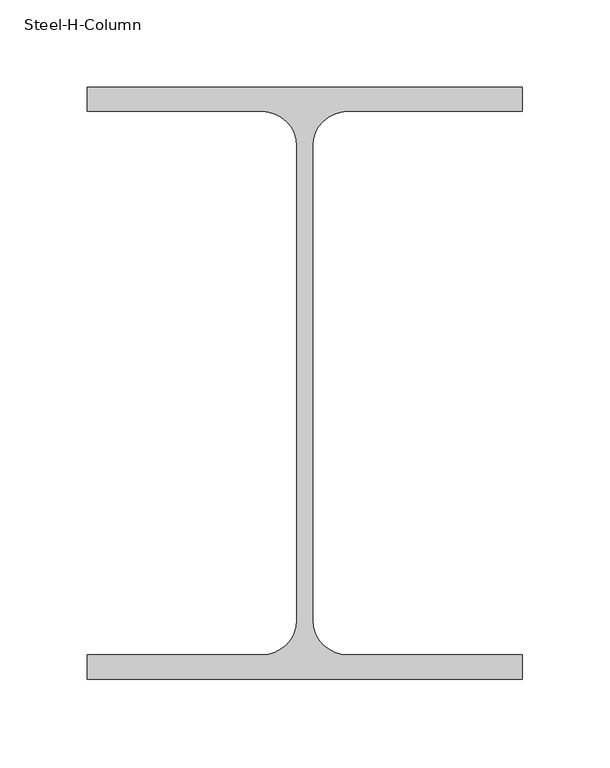
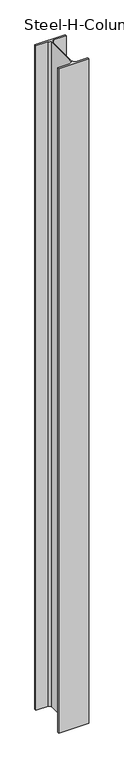
"""IFC4 building model written with IfcOpenShell, lengths in millimetres: column geometry, Steel-H-Column : CL121_H-340×250x9x14."""

from ifc_helpers import new_model, si_unit, point, frame, frame_2d, origin, place, context, project, spatial, polyline, circle_curve, trimmed, segment, composite_curve, outline, extrude, source, transform, mapped, element, save


def steel_h_column_09ca9198(model_context):
    return source(origin(), model_context, "Body", "SweptSolid", [
        extrude(outline(composite_curve([segment(polyline([(125.0, 170.0), (125.0, 156.0), (24.5, 156.0)]), True, "CONTINUOUS"), segment(trimmed(circle_curve(frame_2d((24.5, 136.0)), 20.0), [point((24.5, 156.0))], [point((4.5, 136.0))], True, "CARTESIAN"), True, "CONTINUOUS"), segment(polyline([(4.5, 136.0), (4.5, -136.0)]), True, "CONTINUOUS"), segment(trimmed(circle_curve(frame_2d((24.5, -136.0)), 20.0), [point((4.5, -136.0))], [point((24.5, -156.0))], True, "CARTESIAN"), True, "CONTINUOUS"), segment(polyline([(24.5, -156.0), (125.0, -156.0), (125.0, -170.0), (-125.0, -170.0), (-125.0, -156.0), (-24.5, -156.0)]), True, "CONTINUOUS"), segment(trimmed(circle_curve(frame_2d((-24.5, -136.0)), 20.0), [point((-24.5, -156.0))], [point((-4.5, -136.0))], True, "CARTESIAN"), True, "CONTINUOUS"), segment(polyline([(-4.5, -136.0), (-4.5, 136.0)]), True, "CONTINUOUS"), segment(trimmed(circle_curve(frame_2d((-24.5, 136.0)), 20.0), [point((-4.5, 136.0))], [point((-24.5, 156.0))], True, "CARTESIAN"), True, "CONTINUOUS"), segment(polyline([(-24.5, 156.0), (-125.0, 156.0), (-125.0, 170.0), (125.0, 170.0)]), True, "CONTINUOUS")], self_intersect=False)), frame((0.0, 0.0, 200.0), z_axis=(0.0, 0.0, 1.0), x_axis=(1.0, 0.0, 0.0)), (0.0, 0.0, 1.0), 5800.0),
    ])


if __name__ == "__main__":
    model = new_model("IFC4")
    model_context = context("Model", 3, world=origin())
    ifc_project = project(units=[si_unit("LENGTHUNIT", "METRE", prefix="MILLI")], contexts=[model_context])
    site = spatial("IfcSite", under=ifc_project)
    building = spatial("IfcBuilding", under=site)
    placement = place(None, origin())
    steel_h_column_shape = steel_h_column_09ca9198(model_context)
    element("IfcColumn", 1, ObjectType="Steel-H-Column : CL121_H-340×250x9x14", at=placement, inside=building, context=model_context, shape_type="MappedRepresentation", body=[
        mapped(steel_h_column_shape, transform((0.0, 0.0, 0.0), x_axis=(1.0, 0.0, 0.0), y_axis=(0.0, 1.0, 0.0), z_axis=(0.0, 0.0, 1.0))),
    ])
    save(model, "model.ifc")

# Revit data of these elements
# Type "Steel-H-Column : CL121_H-340×250x9x14"
#   Surface Area = 0.00 m²/m
#   Section Area = 101.5 cm²
#   Mass per Unit Length = 79.70 kg/m
#   B = 250 mm
#   H = 340 mm
#   r = 20 mm
#   tw = 9 mm
#   tf = 14 mm
#   hec_material4 [instance default] = none
#   hec_material2 [instance default] = none
#   hec_material1 [instance default] = none
#   hec_material3 [instance default] = none
#   Structural Material [instance default] = Steel, 45-345
#   Assembly Code = ""
# Element 1 (IfcColumn, "Steel-H-Column : CL121_H-340×250x9x14")
#   hec_material1 = S03AA028-00001_Main Steel Structure Erection Work_Shelter/Building_Medium Steel
#   hec_material3 = F01AC000-00002_Building/Shelter Fire Proofing Work_Intumescent Coating Type_1 hr. rating (UL 1709))
#   Structural Material = S01AA002-00001_Main Steel Structure Fabrication Work_Shelter/Building_Medium Steel - Standard
#   Materials on its faces: "S01AA002-00001_Main Steel Structure Fabrication Work_Shelter/Building_Medium Steel - Standard"
# Materials
#   "Steel, 45-345": class "Metal", colour RGB 189 187 185, transparency 0, Description = "Steel 345 MPa", Cost = 0
#   "S01AA002-00001_Main Steel Structure Fabrication Work_Shelter/Building_Medium Steel - Standard": class "Metal", colour RGB 120 120 120, transparency 0, Comments = "(90KG/M>Weight≥30KG/M)", Description = "Structural steel 50ksi", W00) Work Master Code = "S01AA002-0001", W01) Work Master_Lv1 = "Main Steel Structure Fabrication Work", W02) Work Master_Lv2 = "Shelter/Building", W03) Work Master_Spec.1 = "Medium Steel - Standard (90KG/M>Weight≥30KG/M)", Cost = 0
#   "S03AA028-00001_Main Steel Structure Erection Work_Shelter/Building_Medium Steel": class "Metal", colour RGB 120 120 120, transparency 0, Comments = "(90KG/M>Weight≥30KG/M)", Description = "Structural steel 50ksi", W00) Work Master Code = "S03AA028-0001", W01) Work Master_Lv1 = "Main Steel Structure Erection Work", W02) Work Master_Lv2 = "Shelter/Building", W03) Work Master_Spec.1 = "Medium Steel (90KG/M>Weight≥30KG/M)", Cost = 0
#   "F01AC000-00002_Building/Shelter Fire Proofing Work_Intumescent Coating Type_1 hr. rating (UL 1709))": class "Metal", colour RGB 255 128 128, transparency 0, Description = "Paint finished steel", W00) Work Master Code = "F01AC000-00002", W01) Work Master_Lv1 = "Building/Shelter Fire Proofing Work", W02) Work Master_Lv2 = "Intumescent Coating Type", W03) Work Master_Spec.1 = "1 hr. rating (UL 1709)", Cost = 0
